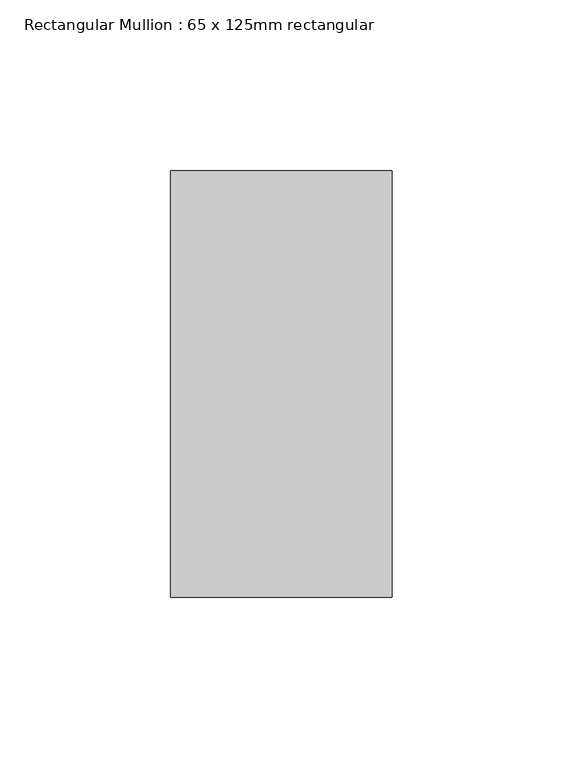
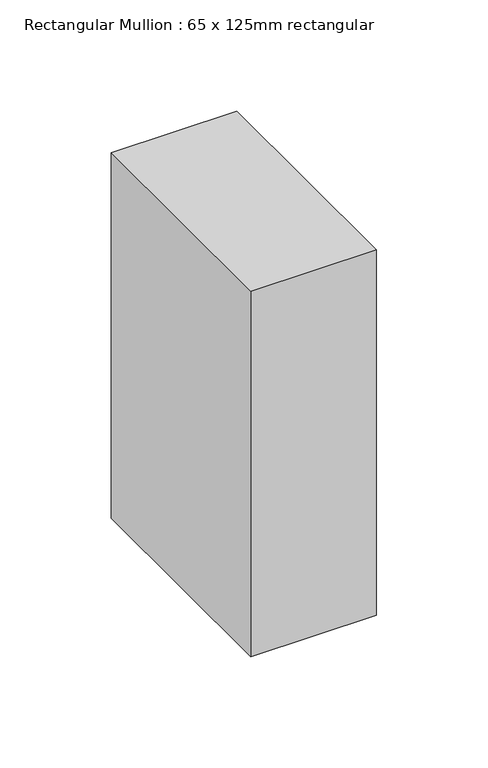
"""IFC4 building model written with IfcOpenShell, lengths in millimetres: member geometry, Rectangular Mullion : 65 x 125mm rectangular."""

from ifc_helpers import new_model, si_unit, frame, origin, place, context, project, spatial, polyline, outline, extrude, source, transform, mapped, element, save


def rectangular_mullion_65_x_125mm_rectangular_dd0f1ba9(model_context):
    return source(origin(), model_context, "Body", "SweptSolid", [
        extrude(outline(polyline([(0.0, 62.5), (0.0, -62.5), (-65.0, -62.5), (-65.0, 62.5), (0.0, 62.5)])), frame((0.0, 0.0, -200.0), z_axis=(0.0, 0.0, 1.0), x_axis=(1.0, 0.0, 0.0)), (0.0, 0.0, 1.0), 200.0),
    ])


if __name__ == "__main__":
    model = new_model("IFC4")
    model_context = context("Model", 3, world=origin())
    ifc_project = project(units=[si_unit("LENGTHUNIT", "METRE", prefix="MILLI")], contexts=[model_context])
    site = spatial("IfcSite", under=ifc_project)
    building = spatial("IfcBuilding", under=site)
    placement = place(None, origin())
    rectangular_mullion_65_x_125mm_rectangular_shape = rectangular_mullion_65_x_125mm_rectangular_dd0f1ba9(model_context)
    element("IfcMember", 1, ObjectType="Rectangular Mullion : 65 x 125mm rectangular", at=placement, inside=building, context=model_context, shape_type="MappedRepresentation", body=[
        mapped(rectangular_mullion_65_x_125mm_rectangular_shape, transform((0.0, 0.0, 0.0), x_axis=(1.0, 0.0, 0.0), y_axis=(0.0, 1.0, 0.0), z_axis=(0.0, 0.0, 1.0))),
    ])
    save(model, "model.ifc")

# Revit data of these elements
# Type "Rectangular Mullion : 65 x 125mm rectangular"
#   built-in parameter 1007304 = 0.410105 (stored number, unit not read)
#   built-in parameter 1007301 = 0.106627 (stored number, unit not read)
#   built-in parameter 1007300 = 0.106627 (stored number, unit not read)
# Element 1 (IfcMember, "Rectangular Mullion : 65 x 125mm rectangular")
#   Materials on its faces: "Aluminum"
# Materials
#   "Aluminum": class "Metal", colour RGB 244 245 246, transparency 0, Description = "Aluminum 6061", Cost = 0
